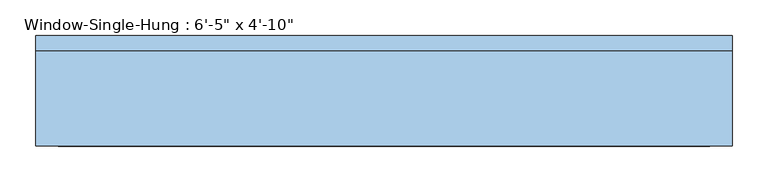
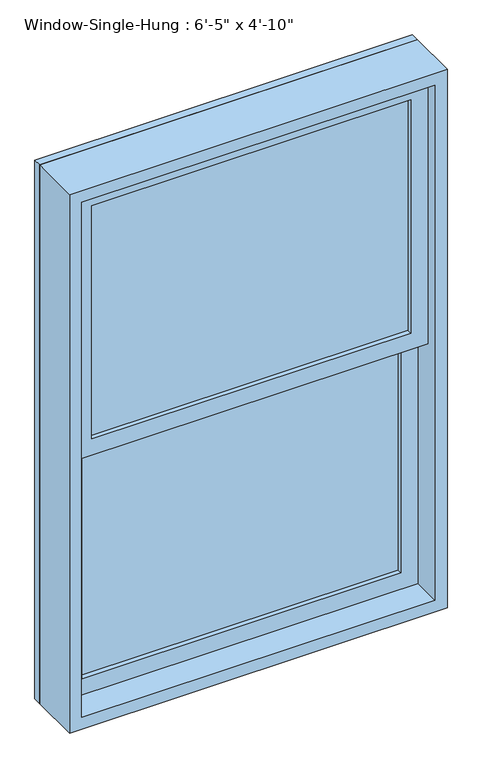
"""IFC4 building model written with IfcOpenShell, lengths in millimetres: window geometry."""

from ifc_helpers import new_model, si_unit, frame, origin, place, context, project, spatial, polyline, outline, extrude, source, transform, mapped, element, save


def window_35671ba8(model_context):
    return source(origin(), model_context, "Body", "SweptSolid", [
        extrude(outline(polyline([(412.75, 1.5875), (-412.75, 1.5875), (-412.75, 7.9375), (412.75, 7.9375), (412.75, 1.5875)])), frame((0.0, 0.0, 990.6), z_axis=(0.0, 0.0, 1.0), x_axis=(1.0, 0.0, 0.0)), (0.0, 0.0, 1.0), 638.175),
        extrude(outline(polyline([(-412.75, 14.2875), (-412.75, 20.6375), (412.75, 20.6375), (412.75, 14.2875), (-412.75, 14.2875)])), frame((0.0, 0.0, 990.6), z_axis=(0.0, 0.0, 1.0), x_axis=(1.0, 0.0, 0.0)), (0.0, 0.0, 1.0), 638.175),
        extrude(outline(polyline([(412.75, -42.8625), (-412.75, -42.8625), (-412.75, -36.5125), (412.75, -36.5125), (412.75, -42.8625)])), frame((0.0, 0.0, 1673.225), z_axis=(0.0, 0.0, 1.0), x_axis=(1.0, 0.0, 0.0)), (0.0, 0.0, 1.0), 638.175),
        extrude(outline(polyline([(-412.75, -30.1625), (-412.75, -23.8125), (412.75, -23.8125), (412.75, -30.1625), (-412.75, -30.1625)])), frame((0.0, 0.0, 1673.225), z_axis=(0.0, 0.0, 1.0), x_axis=(1.0, 0.0, 0.0)), (0.0, 0.0, 1.0), 638.175),
        extrude(outline(polyline([(1673.225, 457.2), (1673.225, -457.2), (946.15, -457.2), (946.15, 457.2), (1673.225, 457.2)]), holes=[polyline([(1628.775, -412.75), (1628.775, 412.75), (990.6, 412.75), (990.6, -412.75), (1628.775, -412.75)])]), frame((0.0, -11.1125, 0.0), z_axis=(0.0, 1.0, 0.0), x_axis=(0.0, 0.0, 1.0)), (0.0, 0.0, 1.0), 44.45),
        extrude(outline(polyline([(2355.85, 457.2), (2355.85, -457.2), (1628.775, -457.2), (1628.775, 457.2), (2355.85, 457.2)]), holes=[polyline([(2311.4, -412.75), (2311.4, 412.75), (1673.225, 412.75), (1673.225, -412.75), (2311.4, -412.75)])]), frame((0.0, -55.5625, 0.0), z_axis=(0.0, 1.0, 0.0), x_axis=(0.0, 0.0, 1.0)), (0.0, 0.0, 1.0), 44.45),
        extrude(outline(polyline([(2387.6, 488.95), (2387.6, -488.95), (914.4, -488.95), (914.4, 488.95), (2387.6, 488.95)]), holes=[polyline([(2355.85, -457.2), (2355.85, 457.2), (946.15, 457.2), (946.15, -457.2), (2355.85, -457.2)])]), frame((0.0, -87.3125, 0.0), z_axis=(0.0, 1.0, 0.0), x_axis=(0.0, 0.0, 1.0)), (0.0, 0.0, 1.0), 133.35),
        extrude(outline(polyline([(2387.6, 488.95), (2387.6, -488.95), (914.4, -488.95), (914.4, 488.95), (2387.6, 488.95)]), holes=[polyline([(2368.55, 469.9), (933.45, 469.9), (933.45, -469.9), (2368.55, -469.9), (2368.55, 469.9)])]), frame((0.0, 46.0375, 0.0), z_axis=(0.0, 1.0, 0.0), x_axis=(0.0, 0.0, 1.0)), (0.0, 0.0, 1.0), 22.225),
    ])


if __name__ == "__main__":
    model = new_model("IFC4")
    model_context = context("Model", 3, world=origin())
    ifc_project = project(units=[si_unit("LENGTHUNIT", "METRE", prefix="MILLI")], contexts=[model_context])
    site = spatial("IfcSite", under=ifc_project)
    building = spatial("IfcBuilding", under=site)
    placement = place(None, origin())
    window_shape = window_35671ba8(model_context)
    element("IfcWindow", 1, ObjectType="Window-Single-Hung : 6'-5\" x 4'-10\"", at=placement, inside=building, context=model_context, shape_type="MappedRepresentation", body=[
        mapped(window_shape, transform((0.0, 0.0, 0.0), x_axis=(1.0, 0.0, 0.0), y_axis=(0.0, 1.0, 0.0), z_axis=(0.0, 0.0, 1.0))),
    ])
    save(model, "model.ifc")

# Revit data of these elements
# Type "Window-Single-Hung : 6'-5\" x 4'-10\""
#   Type Mark = "19"
#   Fire Rating = "0.5h"
#   Construction Type Id = "DG-DR"
#   Assembly Code = "B2020100"
#   Analytic Construction = "Double glazing - domestic"
#   Wall Thickness [instance default] = 0' - 6"
#   Window Inset [instance default] = 0' - 0"
#   Visual Light Transmittance = 0.81
#   Thermal Resistance (R) = 0.319569 (m²·K)/W
#   Solar Heat Gain Coefficient = 0.76
#   Muntin Width = 2' - 8 1/2"
#   Muntin Height = 2' - 1 1/8"
#   Interior Wall Closure [instance default] = 0' - 1 1/2"
#   Rough Width = 3' - 3"
#   Rough Height = 4' - 10 1/2"
#   Frame Extension [instance default] = 0' - 1 1/4"
#   Exterior Wall Closure [instance default] = 0' - 0 1/2"
#   Extension Jamb [instance default] = 0' - 1 1/2"
#   Heat Transfer Coefficient (U) = 3.12929 W/(m²·K)
#   Height = 4' - 10"
#   Width = 3' - 2 1/2"
#   Top Muntin Visibility = yes
#   Indicator Visibility [instance default] = yes
#   Extension Jamb Visibility [instance default] = yes
#   Interior Trim Visibility [instance default] = yes
#   Exterior Trim Visibility [instance default] = yes
#   Bottom Muntin Visibility = yes
#   Muntin Pattern = Muntin Pattern_2x2 : Muntin Pattern_2x2
#   Interior Trim Material = Wood - Stained
#   Interior Trim = Trim-Window-Interior-Flat : Picture Frame
#   Exterior Trim Material = Clad - White
#   Exterior Trim = Trim-Window-Exterior-Flat : with Sill
#   Glass Panel Material = Glass
#   Exterior Frame Material = Clad - White
#   Interior Frame Material = Wood - Stained
#   Wall Closure = (empty or 0)
# Element 1 (IfcWindow, "Window-Single-Hung : 6'-5\" x 4'-10\"")
#   Wall Thickness = 0' - 5 3/8"
#   Extension Jamb = 0' - 0 7/8"
#   Materials on its faces: "Wood - Stained", "Glass", "Clad - White"
# Materials
#   "Wood - Stained": class "Wood", colour RGB 224 178 126, transparency 0, Cost = 0
#   "Clad - White": class "Wood", colour RGB 242 242 238, transparency 0, Cost = 0
#   "Glass": class "Glass", colour RGB 0 128 192, transparency 0.75, Description = "Soda Lime Glass", Cost = 0
